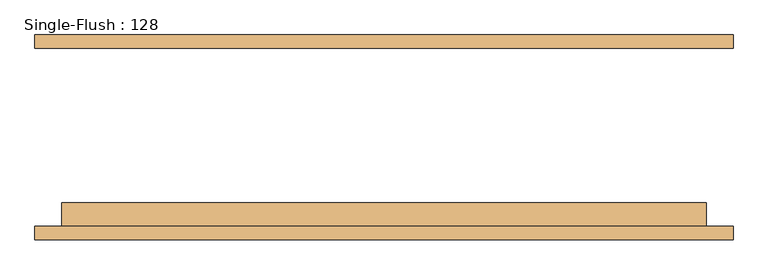
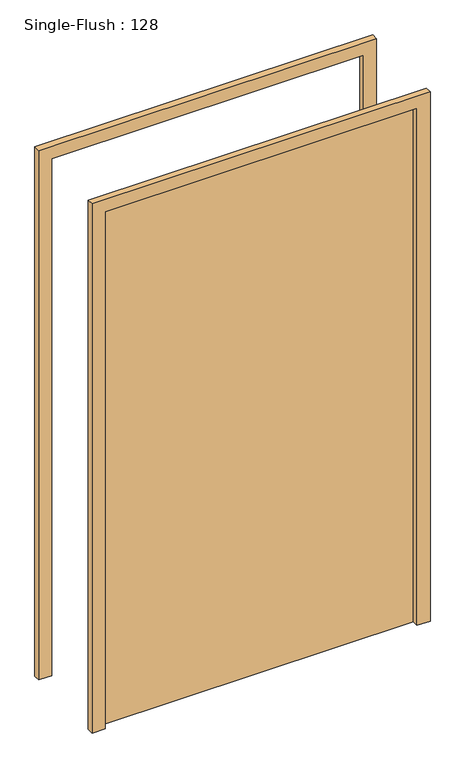
"""IFC4 building model written with IfcOpenShell, lengths in millimetres: door geometry, Single-Flush : 128."""

from ifc_helpers import new_model, si_unit, frame, origin, origin_with_axes, place, context, project, spatial, polyline, outline, extrude, source, transform, mapped, element, save


def single_flush_128_a3bbcc59(model_context):
    return source(origin(), model_context, "Body", "SweptSolid", [
        extrude(outline(polyline([(2184.4, -660.4), (0.0, -660.4), (0.0, -609.6), (2133.6, -609.6), (2133.6, 609.6), (0.0, 609.6), (0.0, 660.4), (2184.4, 660.4), (2184.4, -660.4)])), frame((0.0, -193.675, 0.0), z_axis=(0.0, 1.0, 0.0), x_axis=(0.0, 0.0, 1.0)), (0.0, 0.0, 1.0), 25.4),
        extrude(outline(polyline([(2184.4, 660.4), (2184.4, -660.4), (0.0, -660.4), (0.0, -609.6), (2133.6, -609.6), (2133.6, 609.6), (0.0, 609.6), (0.0, 660.4), (2184.4, 660.4)])), frame((0.0, 168.275, 0.0), z_axis=(0.0, 1.0, 0.0), x_axis=(0.0, 0.0, 1.0)), (0.0, 0.0, 1.0), 25.4),
        extrude(outline(polyline([(609.6, -123.825), (609.6, -168.275), (-609.6, -168.275), (-609.6, -123.825), (609.6, -123.825)])), origin_with_axes(), (0.0, 0.0, 1.0), 2133.6),
    ])


if __name__ == "__main__":
    model = new_model("IFC4")
    model_context = context("Model", 3, world=origin())
    ifc_project = project(units=[si_unit("LENGTHUNIT", "METRE", prefix="MILLI")], contexts=[model_context])
    site = spatial("IfcSite", under=ifc_project)
    building = spatial("IfcBuilding", under=site)
    placement = place(None, origin())
    single_flush_128_shape = single_flush_128_a3bbcc59(model_context)
    element("IfcDoor", 1, ObjectType="Single-Flush : 128", at=placement, inside=building, context=model_context, shape_type="MappedRepresentation", body=[
        mapped(single_flush_128_shape, transform((0.0, 0.0, 0.0), x_axis=(1.0, 0.0, 0.0), y_axis=(0.0, 1.0, 0.0), z_axis=(0.0, 0.0, 1.0))),
    ])
    save(model, "model.ifc")

# Revit data of these elements
# Type "Single-Flush : 128"
#   Type Mark = "128"
#   Construction Type Id = "MDOOR"
#   Assembly Code = "C1020"
#   Analytic Construction = "Metal"
#   Thickness = 0' - 1 3/4"
#   Heat Transfer Coefficient (U) = 3.7021 W/(m²·K)
#   Height = 7' - 0"
#   Trim Projection Ext = 0' - 1"
#   Trim Projection Int = 0' - 1"
#   Trim Width = 0' - 2"
#   Width = 4' - 0"
#   Door Material = 05 - Metal - Steel
#   Frame Material = 05 - Metal - Steel
#   Visual Light Transmittance = 0
#   Solar Heat Gain Coefficient = 0
#   Function = (empty or 0)
#   Wall Closure = (empty or 0)
# Element 1 (IfcDoor, "Single-Flush : 128")
#   Materials on its faces: "05 - Metal - Steel"
# Materials
#   "05 - Metal - Steel": class "Unassigned", colour RGB 199 199 199, transparency 0, Description = "Steel"
